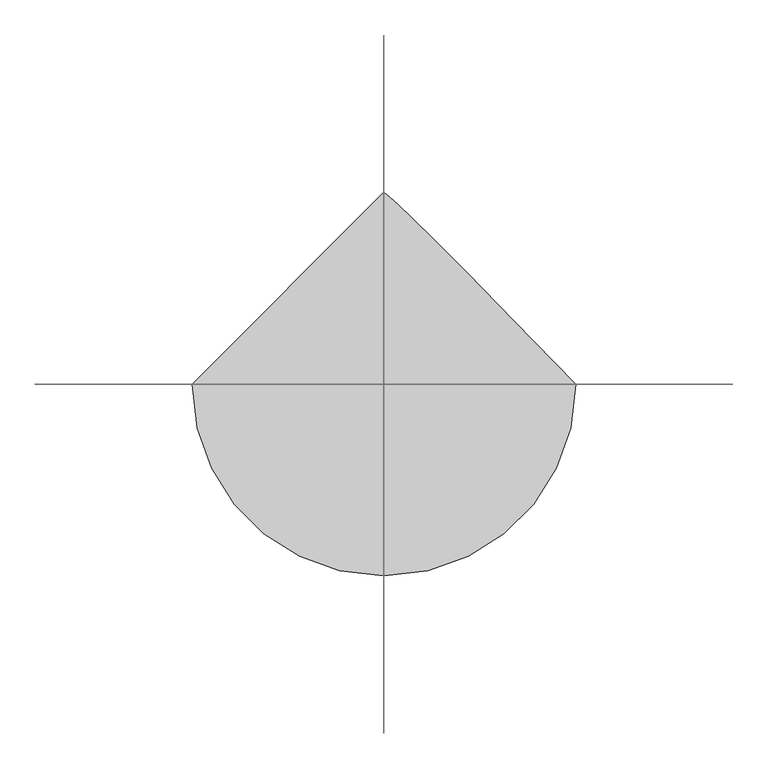
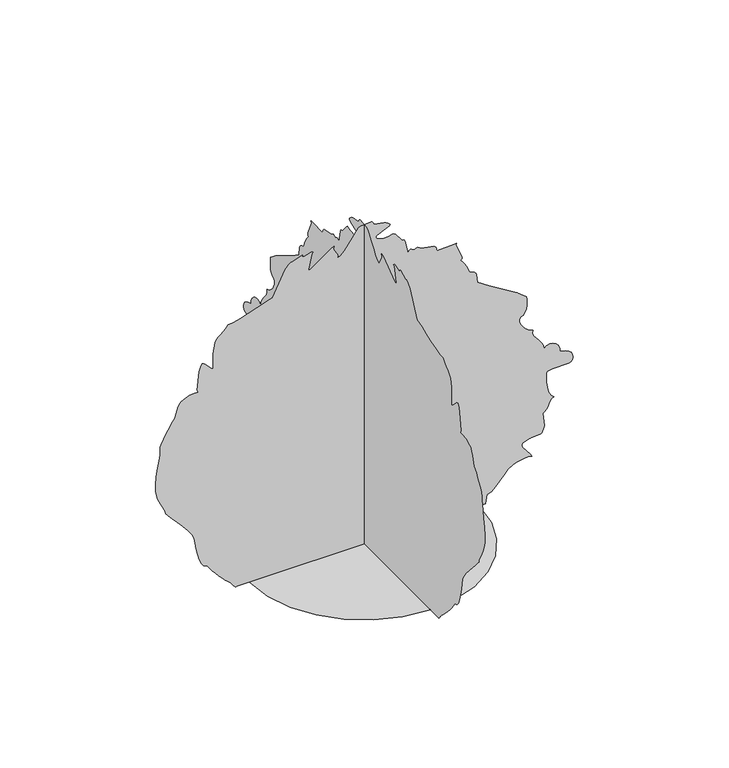
"""IFC4 building model written with IfcOpenShell, lengths in millimetres: proxy geometry, vibernum 26767 : vibernum 26767."""

from ifc_helpers import new_model, si_unit, origin, place, context, project, spatial, triangles, source, transform, mapped, element, save


def entourage_5c4a15e9(model_context):
    return source(origin(), model_context, "Body", "Tessellation", [
        triangles([(-310.4009663, 0.0, 0.0), (-302.1967432, -71.1236111, 0.0), (-278.8261857, -136.4392555, 0.0), (-242.1615087, -194.0757083, 0.0), (-194.0757083, -242.1615087, 0.0), (-136.4392555, -278.8261857, 0.0), (-71.1236111, -302.1967432, 0.0), (1.36e-05, -310.4009663, 0.0), (71.1236111, -302.1967432, 0.0), (136.4392555, -278.8261857, 0.0), (194.0757083, -242.1615087, 0.0), (242.1615087, -194.0757083, 0.0), (278.8261857, -136.4392555, 0.0), (302.1967432, -71.1236111, 0.0), (310.4009663, 2.71e-05, 0.0), (209.5283262, 103.4718092, 0.0), (134.7455816, 179.6535872, 0.0), (81.7052599, 233.0934394, 0.0), (46.0591254, 268.3410517, 0.0), (23.45852, 289.9412231, 0.0), (9.5549798, 302.4456561, 0.0), (-4.07e-05, 310.4009663, 0.0), (-352.7554667, 2.15e-05, 4.3495503), (-355.9965117, 2.13e-05, 8.4826161), (-359.0826241, 2.1e-05, 12.3234041), (-362.0188548, 2.08e-05, 15.7959676), (-364.8077834, 2.07e-05, 18.8245652), (-367.457004, 2.05e-05, 21.3332227), (-369.9665528, 2.04e-05, 23.2460988), (-375.8161594, 2.01e-05, 28.5320975), (-383.5606359, 1.96e-05, 36.3306653), (-392.4582396, 1.9e-05, 45.9079945), (-401.7775108, 1.84e-05, 56.5300297), (-410.7742001, 1.78e-05, 67.463215), (-418.7091808, 1.71e-05, 77.9737471), (-424.8483773, 1.66e-05, 87.3278091), (-434.3200376, 1.64e-05, 90.3102761), (-441.518399, 1.59e-05, 99.1873323), (-446.9133459, 1.51e-05, 112.4136326), (-450.9672046, 1.41e-05, 128.4448579), (-454.1523663, 1.31e-05, 145.7354086), (-456.9311211, 1.21e-05, 162.7404662), (-459.7733894, 1.12e-05, 177.9152122), (-465.8821009, 1.05e-05, 189.8085088), (-476.9463238, 9.6e-06, 205.0848474), (-490.9620744, 8.5e-06, 222.0754346), (-505.927767, 7.5e-06, 239.1112225), (-519.8393452, 6.6e-06, 254.5234358), (-530.6927888, 5.9e-06, 266.6443348), (-536.4840051, 5.5e-06, 273.804599), (-537.980062, 5.1e-06, 279.9056801), (-541.2769901, 4.6e-06, 287.7695352), (-545.6533945, 4.1e-06, 296.6874683), (-550.3904963, 3.6e-06, 305.9584685), (-554.7669371, 3e-06, 314.8764198), (-558.0638288, 2.6e-06, 322.7377496), (-559.5599221, 2.2e-06, 328.8413741), (-564.0633173, 1.1e-06, 346.2505222), (-564.6424607, -1e-07, 367.0963428), (-562.5393188, -1.4e-06, 389.5906094), (-558.9909525, -2.8e-06, 411.9375375), (-555.2393646, -4e-06, 432.3439227), (-552.5215799, -5e-06, 449.0164879), (-552.0770576, -5.6e-06, 460.1619922), (-551.4522048, -6.2e-06, 469.7809908), (-548.1832546, -6.8e-06, 479.8495623), (-543.0422894, -7.4e-06, 490.1772022), (-536.8090942, -8.1e-06, 500.5785295), (-530.2609838, -8.7e-06, 510.8553732), (-524.1776705, -9.2e-06, 520.822352), (-519.3338891, -9.8e-06, 530.2863819), (-514.6958364, -1.01e-05, 534.5764544), (-511.1779552, -1.05e-05, 541.7037083), (-508.3280565, -1.1e-05, 550.5352913), (-505.7042341, -1.16e-05, 559.930757), (-502.8569152, -1.21e-05, 568.7597966), (-499.3364542, -1.25e-05, 575.8870505), (-494.6984015, -1.28e-05, 580.1796301), (-488.7141738, -1.3e-05, 583.3724221), (-483.0575787, -1.32e-05, 586.1308657), (-477.4467293, -1.33e-05, 588.3914835), (-471.5996298, -1.34e-05, 590.0856388), (-465.2318499, -1.35e-05, 591.1448401), (-458.0563431, -1.35e-05, 591.5029578), (-449.7962731, -1.35e-05, 591.0940438), (-452.0898831, -1.38e-05, 597.7844058), (-446.8498687, -1.69e-05, 648.1323137), (-442.8239516, -1.75e-05, 659.7223766), (-438.0639951, -1.8e-05, 668.1551468), (-434.5155925, -1.8e-05, 667.6064884), (-430.9748566, -1.79e-05, 665.0360058), (-414.5257879, -1.68e-05, 647.428723), (-409.2578319, -1.66e-05, 644.4162615), (-408.9962199, -1.74e-05, 657.4007887), (-409.1181238, -1.79e-05, 666.2653639), (-409.3213454, -1.83e-05, 672.7017443), (-409.3035413, -1.87e-05, 678.4040852), (-408.7625133, -1.91e-05, 685.0639257), (-407.3934834, -1.96e-05, 694.3755667), (-404.8915649, -2.04e-05, 708.0306198), (-403.2913719, -2.1e-05, 717.4769182), (-399.8064829, -2.14e-05, 724.3451036), (-394.8255369, -2.17e-05, 729.6460882), (-388.7295427, -2.2e-05, 734.3907841), (-381.9096102, -2.23e-05, 739.5952629), (-374.7468206, -2.27e-05, 746.2703642), (-367.6271971, -2.33e-05, 755.4296162), (-354.5182589, -2.33e-05, 756.2449734), (-335.3386883, -2.36e-05, 761.043009), (-312.9155657, -2.4e-05, 768.2718555), (-290.0885433, -2.45e-05, 776.3821163), (-269.6872632, -2.49e-05, 783.819235), (-254.5437653, -2.53e-05, 789.0313442), (-247.4939957, -2.53e-05, 790.4715179), (-213.6794536, -2.94e-05, 858.769602), (-205.2583288, -3e-05, 869.5493946), (-197.3670409, -3.03e-05, 874.0807314), (-193.2331907, -3.03e-05, 873.8495682), (-168.7295447, -3.09e-05, 884.1188541), (-166.460806, -3.09e-05, 883.4558859), (-168.0742249, -3.06e-05, 879.0896553), (-161.877383, -3.06e-05, 879.3893463), (-144.3734641, -3.09e-05, 884.8376329), (-141.0938133, -3.09e-05, 884.1543898), (-137.9627544, -3.07e-05, 881.4086271), (-140.7920603, -3.07e-05, 880.4332506), (-150.2901451, -2.82e-05, 838.0508085), (-150.4359393, -2.79e-05, 834.0097034), (-142.0369153, -2.81e-05, 837.3624784), (-89.9201382, -3.04e-05, 875.4065952), (-81.5211142, -3.06e-05, 878.7594429), (-83.236371, -3.02e-05, 872.9860308), (-82.0336828, -2.99e-05, 867.6621552), (-72.5891921, -2.9e-05, 852.5922901), (-71.3862495, -2.87e-05, 847.2684872), (-73.1015109, -2.84e-05, 841.495075), (-63.556186, -2.86e-05, 845.6047806), (-53.0855361, -2.92e-05, 856.2092932), (-42.3674857, -3.01e-05, 870.5983858), (-32.0797166, -3.1e-05, 886.0492596), (-22.9007347, -3.19e-05, 899.8541582), (-15.50783, -3.24e-05, 909.2952971), (-10.5790577, -3.25e-05, 911.6575075), (18.9106201, -3.27e-05, 914.4007267), (21.5322068, -3.27e-05, 913.1789989), (23.8564858, -3.25e-05, 909.8845779), (26.6850082, -3.21e-05, 903.8622711), (53.36646, -3.19e-05, 899.8287237), (58.7731068, -3.17e-05, 897.4639698), (63.9669031, -3.15e-05, 893.9232702), (69.0938976, -3.12e-05, 888.8939987), (68.0601171, -3.1e-05, 885.5234196), (63.3263127, -3.08e-05, 882.1706446), (34.7215748, -3.01e-05, 870.0904226), (31.9859905, -2.99e-05, 867.6900604), (32.133565, -2.97e-05, 863.7226427), (35.5686638, -2.95e-05, 860.1538925), (41.5277613, -2.93e-05, 857.2862623), (49.2473392, -2.92e-05, 855.4244574), (57.9630999, -2.92e-05, 854.8808859), (66.9122902, -2.92e-05, 855.9553116), (75.3308715, -2.94e-05, 858.9575993), (79.5358429, -2.94e-05, 858.9905914), (84.1909094, -2.92e-05, 855.1374109), (99.0570351, -2.8e-05, 835.8054514), (103.7123468, -2.78e-05, 831.9522709), (107.9173227, -2.78e-05, 831.9827196), (110.5566329, -2.75e-05, 826.9687815), (117.7400153, -2.54e-05, 791.6018269), (122.069702, -2.57e-05, 796.2169521), (125.2845857, -2.58e-05, 797.6521116), (127.9442162, -2.57e-05, 797.0729319), (133.8415943, -2.56e-05, 794.512623), (138.1999856, -2.56e-05, 794.8580961), (144.2457012, -2.58e-05, 797.8374928), (154.0983702, -2.54e-05, 791.6500797), (188.4892397, -2.5e-05, 784.7844378), (193.5639118, -2.47e-05, 779.5723286), (196.3218285, -2.41e-05, 769.7729994), (243.3426139, -2.42e-05, 771.0379658), (249.3334547, -2.43e-05, 772.2673239), (247.7520468, -2.39e-05, 766.8596598), (263.6852313, -2.17e-05, 729.0644377), (264.3888039, -2.13e-05, 722.3968941), (260.2486133, -2.11e-05, 719.5673429), (264.4396183, -2.09e-05, 715.6404751), (268.5899827, -2.05e-05, 710.080422), (272.58794, -2.02e-05, 703.4306826), (276.3268288, -1.97e-05, 696.2399878), (279.6948645, -1.93e-05, 689.0492203), (282.5828423, -1.89e-05, 682.4020243), (284.8815392, -1.86e-05, 676.8470581), (292.1535699, -1.84e-05, 674.5203833), (297.5205933, -1.82e-05, 671.6629269), (301.2772681, -1.8e-05, 668.0231054), (303.7181983, -1.78e-05, 663.3520243), (306.0880391, -1.64e-05, 640.6748474), (337.5484735, -1.51e-05, 619.285528), (412.8366832, -1.23e-05, 572.7882208), (438.1198783, -1.12e-05, 553.4791523), (439.8826341, -1.08e-05, 546.9589471), (439.9893136, -9.7e-06, 528.3128105), (438.1224217, -9.1e-06, 518.4956772), (434.833124, -8.6e-06, 509.8850836), (430.0172479, -8.2e-06, 503.634157), (423.57073, -8.1e-06, 500.8960247), (419.6083265, -7.7e-06, 495.2673712), (419.9613936, -7.3e-06, 487.2053996), (423.7561475, -6.7e-06, 477.8835849), (430.1112465, -6.1e-06, 468.4703513), (438.1503633, -5.6e-06, 460.136594), (446.9946273, -5.3e-06, 454.0533171), (455.7652765, -5.1e-06, 451.3913793), (454.5663671, -4.6e-06, 443.4767461), (457.9420332, -4.1e-06, 435.1353584), (464.2260246, -3.6e-06, 426.3952306), (471.7495116, -3.1e-06, 417.2791446), (478.8462805, -2.5e-06, 407.8151147), (483.8449943, -1.9e-06, 398.025923), (485.0794393, -1.3e-06, 387.9344968), (492.6181506, -1.7e-06, 394.3632468), (501.3405107, -1.8e-06, 396.5095548), (510.2914905, -1.8e-06, 394.9982735), (518.5109379, -1.5e-06, 390.4541831), (525.0463675, -1.1e-06, 383.5047526), (528.9401705, -5e-07, 374.7773057), (529.2322675, 0.0, 364.8966951), (543.28359, 2e-07, 361.6200783), (553.2505325, 5e-07, 356.9591709), (559.7300789, 8e-07, 351.3864369), (563.3267344, 1.2e-06, 345.3742312), (564.6424607, 1.5e-06, 339.3975975), (564.2741693, 1.9e-06, 333.9264562), (562.8263652, 2.1e-06, 329.438249), (558.5058077, 2.4e-06, 325.0237292), (551.6808246, 2.5e-06, 323.3371679), (508.3052018, 2.5e-06, 323.4667022), (495.6814084, 2.7e-06, 320.1113837), (493.0550426, 3e-06, 315.2853702), (491.9247336, 3.6e-06, 304.683401), (492.3870237, 4.5e-06, 290.5000371), (494.5434691, 5.4e-06, 274.934908), (498.4855614, 6.3e-06, 260.1850997), (504.3148567, 7e-06, 248.4462268), (512.1304407, 7.4e-06, 241.918682), (506.1944658, 7.6e-06, 237.9293542), (502.0110729, 7.9e-06, 232.375896), (498.8894248, 8.3e-06, 225.9143899), (496.1360682, 8.7e-06, 219.2011551), (493.06518, 9.1e-06, 212.8918018), (488.9859595, 9.4e-06, 207.6423766), (483.2074605, 9.6e-06, 204.1089804), (486.5094392, 1.18e-05, 167.9235982), (484.7949363, 1.23e-05, 159.1671923), (479.7174846, 1.29e-05, 149.4257811), (478.0410971, 1.3e-05, 147.3986065), (448.2189348, 1.31e-05, 145.3638107), (427.0784738, 1.35e-05, 138.6241693), (425.673872, 1.39e-05, 132.82763), (427.5890167, 1.42e-05, 126.7778539), (449.1968184, 1.58e-05, 99.5421708), (453.2709884, 1.63e-05, 91.8492719), (446.9844898, 1.62e-05, 94.1108889), (432.729982, 1.62e-05, 94.2706539), (416.3113984, 1.64e-05, 90.1472137), (414.6045259, 1.65e-05, 89.3547294), (401.3177642, 1.66e-05, 85.9130245), (388.9555827, 1.72e-05, 76.9775597), (377.2588766, 1.79e-05, 64.7009653), (365.9660339, 1.87e-05, 51.235649), (354.8103559, 1.95e-05, 38.7350312), (343.5327375, 2e-05, 29.3512471), (331.8716034, 2.03e-05, 25.2371292), (326.9541347, 2.18e-05, 4e-05), (-349.3544025, 2.18e-05, 4e-05), (-4.6e-06, -352.7554667, 4.3495758), (-4.6e-06, -355.9965117, 8.4826416), (-4.6e-06, -359.0826241, 12.3234041), (-4.6e-06, -362.0188548, 15.7959937), (-4.6e-06, -364.8077834, 18.8245902), (-4.6e-06, -367.457004, 21.3332477), (-4.6e-06, -369.9665528, 23.2460988), (-4.6e-06, -375.8161594, 28.5320975), (-4.6e-06, -383.5606359, 36.3306653), (-4.6e-06, -392.4582396, 45.9079945), (-4.6e-06, -401.7775108, 56.5300297), (-4.6e-06, -410.7742001, 67.4634693), (-4.6e-06, -418.7091808, 77.9737471), (-4.6e-06, -424.8483773, 87.3278091), (-4.6e-06, -434.3200376, 90.3102761), (-4.6e-06, -441.518399, 99.1873323), (-4.6e-06, -446.9133459, 112.4138869), (-4.6e-06, -450.9672046, 128.4448579), (-4.6e-06, -454.1523663, 145.7354086), (-4.6e-06, -456.9311211, 162.7404662), (-4.6e-06, -459.7733894, 177.9152122), (-4.6e-06, -465.8821009, 189.8085088), (-4.6e-06, -476.9463238, 205.0848474), (-4.6e-06, -490.9620744, 222.0754346), (-4.6e-06, -505.927767, 239.1112225), (-4.6e-06, -519.8393452, 254.5234358), (-4.6e-06, -530.6927888, 266.6443348), (-4.6e-06, -536.4840051, 273.804599), (-4.6e-06, -537.980062, 279.9056801), (-4.6e-06, -541.2769901, 287.7695352), (-4.6e-06, -545.6533945, 296.6874683), (-4.6e-06, -550.3904963, 305.9584685), (-4.6e-06, -554.7669371, 314.8764198), (-4.6e-06, -558.0638288, 322.7377496), (-4.6e-06, -559.5599221, 328.8413741), (-4.6e-06, -564.0633173, 346.2505222), (-4.6e-06, -564.6424607, 367.0963428), (-4.6e-06, -562.5393188, 389.5906094), (-4.6e-06, -558.9909525, 411.9375375), (-4.6e-06, -555.2393646, 432.3439227), (-4.6e-06, -552.5215799, 449.0164879), (-4.6e-06, -552.0770576, 460.1619922), (-4.6e-06, -551.4522048, 469.7809908), (-4.6e-06, -548.1832546, 479.8495623), (-4.6e-06, -543.0422894, 490.1772022), (-4.6e-06, -536.8090942, 500.5785295), (-4.6e-06, -530.2609838, 510.8553732), (-4.6e-06, -524.1776705, 520.822352), (-4.6e-06, -519.3338891, 530.2863819), (-4.6e-06, -514.6958364, 534.5764544), (-4.6e-06, -511.1779552, 541.7037083), (-4.6e-06, -508.3280565, 550.5352913), (-4.6e-06, -505.7042341, 559.930757), (-4.6e-06, -502.8569152, 568.7597966), (-4.6e-06, -499.3364542, 575.889594), (-4.6e-06, -494.6984015, 580.1796301), (-4.6e-06, -488.7141738, 583.3724221), (-4.6e-06, -483.0575787, 586.1308657), (-4.6e-06, -477.4467293, 588.3914835), (-4.6e-06, -471.5996298, 590.0856388), (-4.6e-06, -465.2318499, 591.1448401), (-4.6e-06, -458.0563431, 591.5029578), (-4.6e-06, -449.7962731, 591.0940438), (-4.6e-06, -452.0898831, 597.7844058), (-4.6e-06, -446.8498687, 648.1323137), (-4.6e-06, -442.8239516, 659.7223766), (-4.6e-06, -438.0639951, 668.1551468), (-4.6e-06, -434.5155925, 667.6064884), (-4.6e-06, -430.9748566, 665.0360058), (-4.6e-06, -414.5257879, 647.428723), (-4.6e-06, -409.2578319, 644.4162615), (-4.6e-06, -408.9962199, 657.4007887), (-4.6e-06, -409.1181238, 666.2653639), (-4.6e-06, -409.3213454, 672.7017443), (-4.6e-06, -409.3035413, 678.4040852), (-4.6e-06, -408.7625133, 685.0639257), (-4.6e-06, -407.3934834, 694.3755667), (-4.6e-06, -404.8915649, 708.0306198), (-4.6e-06, -403.2913719, 717.4769182), (-4.6e-06, -399.8064829, 724.3451036), (-4.6e-06, -394.8255369, 729.6460882), (-4.6e-06, -388.7295427, 734.3907841), (-4.6e-06, -381.9096102, 739.5952629), (-4.6e-06, -374.7468206, 746.2703642), (-4.6e-06, -367.6271971, 755.4296162), (-4.6e-06, -354.5182589, 756.2449734), (-4.6e-06, -335.3386883, 761.043009), (-4.6e-06, -312.9155657, 768.2718555), (-4.6e-06, -290.0885433, 776.3821163), (-4.6e-06, -269.6872632, 783.819235), (-4.6e-06, -254.5437653, 789.0313442), (-4.6e-06, -247.4939957, 790.4715179), (-4.6e-06, -213.6794536, 858.769602), (-4.6e-06, -205.2583288, 869.5493946), (-4.6e-06, -197.3670409, 874.0807314), (-4.6e-06, -193.2331907, 873.8495682), (-4.6e-06, -168.7295447, 884.1188541), (-4.6e-06, -166.4605516, 883.4558859), (-4.6e-06, -168.0742249, 879.0896553), (-4.6e-06, -161.877383, 879.3893463), (-4.6e-06, -144.3734641, 884.8376329), (-4.6e-06, -141.0938133, 884.1543898), (-4.6e-06, -137.9627544, 881.4086271), (-4.6e-06, -140.7920603, 880.4332506), (-4.6e-06, -150.2901451, 838.0508085), (-4.6e-06, -150.4359393, 834.0121742), (-4.6e-06, -142.0369153, 837.3624784), (-4.6e-06, -89.9201382, 875.4065952), (-4.6e-06, -81.5211142, 878.7594429), (-4.6e-06, -83.236371, 872.9860308), (-4.6e-06, -82.0336828, 867.6621552), (-4.6e-06, -72.5891921, 852.5922901), (-4.6e-06, -71.3862495, 847.2684872), (-4.6e-06, -73.1015109, 841.495075), (-4.6e-06, -63.556186, 845.6047806), (-4.6e-06, -53.0855361, 856.2092932), (-4.6e-06, -42.3674857, 870.5983858), (-4.6e-06, -32.0797166, 886.0492596), (-4.6e-06, -22.9007347, 899.8541582), (-4.6e-06, -15.50783, 909.2952971), (-4.6e-06, -10.5790577, 911.6575075), (-4.6e-06, 18.9106201, 914.4007267), (-4.6e-06, 21.5322068, 913.1789989), (-4.6e-06, 23.8564858, 909.8845779), (-4.6e-06, 26.6850082, 903.8622711), (-4.6e-06, 53.36646, 899.8287237), (-4.6e-06, 58.7731068, 897.4639698), (-4.6e-06, 63.9669031, 893.9232702), (-4.6e-06, 69.0938976, 888.8939987), (-4.6e-06, 68.0601171, 885.5234196), (-4.6e-06, 63.3263127, 882.173188), (-4.6e-06, 34.7215748, 870.0904226), (-4.6e-06, 31.9859905, 867.6900604), (-4.6e-06, 32.133565, 863.7226427), (-4.6e-06, 35.5686638, 860.1538925), (-4.6e-06, 41.5277613, 857.2862623), (-4.6e-06, 49.2473392, 855.4269281), (-4.6e-06, 57.9630999, 854.8808859), (-4.6e-06, 66.9122902, 855.9553116), (-4.6e-06, 75.3308715, 858.9575993), (-4.6e-06, 79.5358429, 858.9905914), (-4.6e-06, 84.1909094, 855.1374109), (-4.6e-06, 99.0570351, 835.8054514), (-4.6e-06, 103.7123468, 831.9522709), (-4.6e-06, 107.9173227, 831.9852631), (-4.6e-06, 110.5566329, 826.9687815), (-4.6e-06, 117.7400153, 791.6018269), (-4.6e-06, 122.069702, 796.2169521), (-4.6e-06, 125.2845857, 797.6521116), (-4.6e-06, 127.9442162, 797.0729319), (-4.6e-06, 133.8415943, 794.512623), (-4.6e-06, 138.1999856, 794.8580961), (-4.6e-06, 144.2457012, 797.8374928), (-4.6e-06, 154.0983702, 791.6500797), (-4.6e-06, 188.4892397, 784.7844378), (-4.6e-06, 193.5639118, 779.5723286), (-4.6e-06, 196.3218285, 769.7729994), (-4.6e-06, 243.3426139, 771.0379658), (-4.6e-06, 249.3334547, 772.2673239), (-4.6e-06, 247.7520468, 766.8596598), (-4.6e-06, 263.6852313, 729.0644377), (-4.6e-06, 264.3888039, 722.3968941), (-4.6e-06, 260.2486133, 719.5673429), (-4.6e-06, 264.4396183, 715.6404751), (-4.6e-06, 268.5899827, 710.080422), (-4.6e-06, 272.58794, 703.4306826), (-4.6e-06, 276.3268288, 696.2399878), (-4.6e-06, 279.6948645, 689.0492203), (-4.6e-06, 282.5828423, 682.4020243), (-4.6e-06, 284.8815392, 676.8470581), (-4.6e-06, 292.1535699, 674.5203833), (-4.6e-06, 297.5205933, 671.6629269), (-4.6e-06, 301.2772681, 668.0231054), (-4.6e-06, 303.7181983, 663.3520243), (-4.6e-06, 306.0880391, 640.6748474), (-4.6e-06, 337.5484735, 619.285528), (-4.6e-06, 412.8366832, 572.7907642), (-4.6e-06, 438.1198783, 553.4791523), (-4.6e-06, 439.8826341, 546.9589471), (-4.6e-06, 439.9893136, 528.3128105), (-4.6e-06, 438.1224217, 518.4956772), (-4.6e-06, 434.833124, 509.8850836), (-4.6e-06, 430.0172479, 503.634157), (-4.6e-06, 423.57073, 500.8960247), (-4.6e-06, 419.6083265, 495.2673712), (-4.6e-06, 419.9613936, 487.2053996), (-4.6e-06, 423.7561475, 477.8835849), (-4.6e-06, 430.1112465, 468.4703513), (-4.6e-06, 438.1503633, 460.136594), (-4.6e-06, 446.9946273, 454.0533171), (-4.6e-06, 455.7652765, 451.3913793), (-4.6e-06, 454.5663671, 443.4767461), (-4.6e-06, 457.9420332, 435.1353584), (-4.6e-06, 464.2260246, 426.3952306), (-4.6e-06, 471.7495116, 417.2791446), (-4.6e-06, 478.8462805, 407.8151147), (-4.6e-06, 483.8449943, 398.025923), (-4.6e-06, 485.0794393, 387.9344968), (-4.6e-06, 492.6181506, 394.3632468), (-4.6e-06, 501.3405107, 396.5095548), (-4.6e-06, 510.2914905, 394.9982735), (-4.6e-06, 518.5109379, 390.4541831), (-4.6e-06, 525.0463675, 383.5047526), (-4.6e-06, 528.9401705, 374.7773057), (-4.6e-06, 529.2322675, 364.8966951), (-4.6e-06, 543.28359, 361.6200783), (-4.6e-06, 553.2505325, 356.9591709), (-4.6e-06, 559.7300789, 351.3864369), (-4.6e-06, 563.3267344, 345.3742312), (-4.6e-06, 564.6424607, 339.3975975), (-4.6e-06, 564.2741693, 333.9264562), (-4.6e-06, 562.8263652, 329.438249), (-4.6e-06, 558.5058077, 325.0237292), (-4.6e-06, 551.6808246, 323.3371679), (-4.6e-06, 508.3052018, 323.4667022), (-4.6e-06, 495.6814084, 320.1113837), (-4.6e-06, 493.0550426, 315.2853702), (-4.6e-06, 491.9247336, 304.683401), (-4.6e-06, 492.3870237, 290.5000371), (-4.6e-06, 494.5434691, 274.934908), (-4.6e-06, 498.4855614, 260.1850997), (-4.6e-06, 504.3148567, 248.4464812), (-4.6e-06, 512.1304407, 241.918682), (-4.6e-06, 506.1944658, 237.9293542), (-4.6e-06, 502.0110729, 232.375896), (-4.6e-06, 498.8894248, 225.9143899), (-4.6e-06, 496.1360682, 219.2011551), (-4.6e-06, 493.06518, 212.8918018), (-4.6e-06, 488.9859595, 207.6423766), (-4.6e-06, 483.2074605, 204.1089804), (-4.6e-06, 486.5094392, 167.9235982), (-4.6e-06, 484.7949363, 159.1671923), (-4.6e-06, 479.7174846, 149.4257811), (-4.6e-06, 478.0410971, 147.3988609), (-4.6e-06, 448.2189348, 145.3638107), (-4.6e-06, 427.0784738, 138.6241693), (-4.6e-06, 425.673872, 132.8278843), (-4.6e-06, 427.5890167, 126.7778539), (-4.6e-06, 449.1968184, 99.5421708), (-4.6e-06, 453.2709884, 91.8492719), (-4.6e-06, 446.9844898, 94.1108889), (-4.6e-06, 432.729982, 94.2706539), (-4.6e-06, 416.3113984, 90.1472137), (-4.6e-06, 414.6045259, 89.3547294), (-4.6e-06, 401.3177642, 85.9130245), (-4.6e-06, 388.9555827, 76.9775597), (-4.6e-06, 377.2588766, 64.7009653), (-4.6e-06, 365.9660339, 51.235649), (-4.6e-06, 354.8103559, 38.7350312), (-4.6e-06, 343.5327375, 29.3512471), (-4.6e-06, 331.8716034, 25.2371564), (-4.6e-06, 326.9541347, 6.03e-05), (-4.6e-06, -349.3544025, 6.03e-05)], [[21, 22, 1], [20, 21, 1], [19, 20, 1], [18, 19, 1], [17, 18, 1], [17, 1, 2], [17, 2, 3], [17, 3, 4], [16, 17, 4], [16, 4, 5], [16, 5, 6], [16, 6, 7], [16, 7, 8], [16, 8, 9], [16, 9, 10], [16, 10, 11], [16, 11, 12], [15, 16, 12], [14, 15, 12], [13, 14, 12], [261, 262, 263], [130, 131, 132], [124, 125, 126], [180, 181, 182], [244, 245, 246], [119, 120, 121], [118, 119, 121], [212, 213, 214], [273, 274, 275], [123, 124, 126], [260, 261, 263], [88, 89, 90], [88, 90, 91], [260, 263, 264], [87, 88, 91], [87, 91, 92], [122, 123, 126], [166, 167, 168], [150, 151, 152], [150, 152, 153], [149, 150, 153], [148, 149, 153], [148, 153, 154], [147, 148, 154], [147, 154, 155], [87, 92, 93], [183, 184, 185], [122, 126, 127], [121, 122, 127], [174, 175, 176], [130, 132, 133], [129, 130, 133], [260, 264, 265], [129, 133, 134], [129, 134, 135], [129, 135, 136], [273, 275, 23], [86, 87, 93], [85, 86, 93], [273, 23, 24], [273, 24, 25], [273, 25, 26], [118, 121, 127], [118, 127, 128], [106, 107, 108], [273, 26, 27], [260, 265, 266], [260, 266, 267], [259, 260, 267], [244, 246, 247], [179, 180, 182], [273, 27, 28], [255, 256, 257], [162, 163, 164], [161, 162, 164], [117, 118, 128], [116, 117, 128], [115, 116, 128], [114, 115, 128], [273, 28, 29], [273, 29, 30], [273, 30, 31], [273, 31, 32], [273, 32, 33], [273, 33, 34], [273, 34, 35], [273, 35, 36], [161, 164, 165], [170, 171, 172], [169, 170, 172], [169, 172, 173], [254, 255, 257], [253, 254, 257], [252, 253, 257], [252, 257, 258], [243, 244, 247], [160, 161, 165], [36, 37, 38], [243, 247, 248], [36, 38, 39], [273, 36, 39], [273, 39, 40], [273, 40, 41], [273, 41, 42], [273, 42, 43], [273, 43, 44], [273, 44, 45], [273, 45, 46], [273, 46, 47], [272, 273, 47], [271, 272, 47], [270, 271, 47], [269, 270, 47], [268, 269, 47], [267, 268, 47], [259, 267, 47], [258, 259, 47], [252, 258, 47], [252, 47, 48], [252, 48, 49], [252, 49, 50], [252, 50, 51], [252, 51, 52], [252, 52, 53], [252, 53, 54], [252, 54, 55], [252, 55, 56], [252, 56, 57], [252, 57, 58], [252, 58, 59], [252, 59, 60], [252, 60, 61], [252, 61, 62], [252, 62, 63], [252, 63, 64], [252, 64, 65], [252, 65, 66], [252, 66, 67], [252, 67, 68], [252, 68, 69], [252, 69, 70], [252, 70, 71], [252, 71, 72], [252, 72, 73], [252, 73, 74], [252, 74, 75], [252, 75, 76], [252, 76, 77], [252, 77, 78], [252, 78, 79], [252, 79, 80], [252, 80, 81], [252, 81, 82], [252, 82, 83], [252, 83, 84], [252, 84, 85], [252, 85, 93], [252, 93, 94], [252, 94, 95], [252, 95, 96], [252, 96, 97], [252, 97, 98], [252, 98, 99], [252, 99, 100], [252, 100, 101], [252, 101, 102], [252, 102, 103], [252, 103, 104], [252, 104, 105], [252, 105, 106], [252, 106, 108], [252, 108, 109], [252, 109, 110], [252, 110, 111], [252, 111, 112], [252, 112, 113], [252, 113, 114], [252, 114, 128], [252, 128, 129], [252, 129, 136], [252, 136, 137], [252, 137, 138], [251, 252, 138], [250, 251, 138], [249, 250, 138], [248, 249, 138], [243, 248, 138], [242, 243, 138], [241, 242, 138], [240, 241, 138], [239, 240, 138], [238, 239, 138], [238, 138, 139], [238, 139, 140], [238, 140, 141], [238, 141, 142], [238, 142, 143], [237, 238, 143], [234, 235, 236], [233, 234, 236], [232, 233, 236], [231, 232, 236], [230, 231, 236], [229, 230, 236], [228, 229, 236], [227, 228, 236], [227, 236, 237], [179, 182, 183], [179, 183, 185], [199, 200, 201], [199, 201, 202], [199, 202, 203], [199, 203, 204], [199, 204, 205], [199, 205, 206], [199, 206, 207], [198, 199, 207], [198, 207, 208], [144, 145, 146], [144, 146, 147], [144, 147, 155], [143, 144, 155], [143, 155, 156], [237, 143, 156], [237, 156, 157], [237, 157, 158], [237, 158, 159], [237, 159, 160], [177, 178, 179], [226, 227, 237], [225, 226, 237], [224, 225, 237], [223, 224, 237], [222, 223, 237], [221, 222, 237], [220, 221, 237], [220, 237, 160], [219, 220, 160], [218, 219, 160], [166, 168, 169], [165, 166, 169], [160, 165, 169], [218, 160, 169], [217, 218, 169], [216, 217, 169], [215, 216, 169], [215, 169, 173], [215, 173, 174], [215, 174, 176], [211, 212, 214], [211, 214, 215], [194, 195, 196], [193, 194, 196], [192, 193, 196], [192, 196, 197], [197, 198, 208], [176, 177, 179], [197, 208, 209], [176, 179, 185], [185, 186, 187], [176, 185, 187], [176, 187, 188], [176, 188, 189], [176, 189, 190], [176, 190, 191], [176, 191, 192], [176, 192, 197], [176, 197, 209], [176, 209, 210], [215, 176, 210], [211, 215, 210], [514, 515, 516], [383, 384, 385], [377, 378, 379], [433, 434, 435], [497, 498, 499], [372, 373, 374], [371, 372, 374], [465, 466, 467], [526, 527, 528], [376, 377, 379], [513, 514, 516], [341, 342, 343], [341, 343, 344], [513, 516, 517], [340, 341, 344], [340, 344, 345], [375, 376, 379], [419, 420, 421], [403, 404, 405], [403, 405, 406], [402, 403, 406], [401, 402, 406], [401, 406, 407], [400, 401, 407], [400, 407, 408], [340, 345, 346], [436, 437, 438], [375, 379, 380], [374, 375, 380], [427, 428, 429], [383, 385, 386], [382, 383, 386], [513, 517, 518], [382, 386, 387], [382, 387, 388], [382, 388, 389], [526, 528, 276], [339, 340, 346], [338, 339, 346], [526, 276, 277], [526, 277, 278], [526, 278, 279], [371, 374, 380], [371, 380, 381], [359, 360, 361], [526, 279, 280], [513, 518, 519], [513, 519, 520], [512, 513, 520], [497, 499, 500], [432, 433, 435], [526, 280, 281], [508, 509, 510], [415, 416, 417], [414, 415, 417], [370, 371, 381], [369, 370, 381], [368, 369, 381], [367, 368, 381], [526, 281, 282], [526, 282, 283], [526, 283, 284], [526, 284, 285], [526, 285, 286], [526, 286, 287], [526, 287, 288], [526, 288, 289], [414, 417, 418], [423, 424, 425], [422, 423, 425], [422, 425, 426], [507, 508, 510], [506, 507, 510], [505, 506, 510], [505, 510, 511], [496, 497, 500], [413, 414, 418], [289, 290, 291], [496, 500, 501], [289, 291, 292], [526, 289, 292], [526, 292, 293], [526, 293, 294], [526, 294, 295], [526, 295, 296], [526, 296, 297], [526, 297, 298], [526, 298, 299], [526, 299, 300], [525, 526, 300], [524, 525, 300], [523, 524, 300], [522, 523, 300], [521, 522, 300], [520, 521, 300], [512, 520, 300], [511, 512, 300], [505, 511, 300], [505, 300, 301], [505, 301, 302], [505, 302, 303], [505, 303, 304], [505, 304, 305], [505, 305, 306], [505, 306, 307], [505, 307, 308], [505, 308, 309], [505, 309, 310], [505, 310, 311], [505, 311, 312], [505, 312, 313], [505, 313, 314], [505, 314, 315], [505, 315, 316], [505, 316, 317], [505, 317, 318], [505, 318, 319], [505, 319, 320], [505, 320, 321], [505, 321, 322], [505, 322, 323], [505, 323, 324], [505, 324, 325], [505, 325, 326], [505, 326, 327], [505, 327, 328], [505, 328, 329], [505, 329, 330], [505, 330, 331], [505, 331, 332], [505, 332, 333], [505, 333, 334], [505, 334, 335], [505, 335, 336], [505, 336, 337], [505, 337, 338], [505, 338, 346], [505, 346, 347], [505, 347, 348], [505, 348, 349], [505, 349, 350], [505, 350, 351], [505, 351, 352], [505, 352, 353], [505, 353, 354], [505, 354, 355], [505, 355, 356], [505, 356, 357], [505, 357, 358], [505, 358, 359], [505, 359, 361], [505, 361, 362], [505, 362, 363], [505, 363, 364], [505, 364, 365], [505, 365, 366], [505, 366, 367], [505, 367, 381], [505, 381, 382], [505, 382, 389], [505, 389, 390], [505, 390, 391], [504, 505, 391], [503, 504, 391], [502, 503, 391], [501, 502, 391], [496, 501, 391], [495, 496, 391], [494, 495, 391], [493, 494, 391], [492, 493, 391], [491, 492, 391], [491, 391, 392], [491, 392, 393], [491, 393, 394], [491, 394, 395], [491, 395, 396], [490, 491, 396], [487, 488, 489], [486, 487, 489], [485, 486, 489], [484, 485, 489], [483, 484, 489], [482, 483, 489], [481, 482, 489], [480, 481, 489], [480, 489, 490], [432, 435, 436], [432, 436, 438], [452, 453, 454], [452, 454, 455], [452, 455, 456], [452, 456, 457], [452, 457, 458], [452, 458, 459], [452, 459, 460], [451, 452, 460], [451, 460, 461], [397, 398, 399], [397, 399, 400], [397, 400, 408], [396, 397, 408], [396, 408, 409], [490, 396, 409], [490, 409, 410], [490, 410, 411], [490, 411, 412], [490, 412, 413], [430, 431, 432], [479, 480, 490], [478, 479, 490], [477, 478, 490], [476, 477, 490], [475, 476, 490], [474, 475, 490], [473, 474, 490], [473, 490, 413], [472, 473, 413], [471, 472, 413], [419, 421, 422], [418, 419, 422], [413, 418, 422], [471, 413, 422], [470, 471, 422], [469, 470, 422], [468, 469, 422], [468, 422, 426], [468, 426, 427], [468, 427, 429], [464, 465, 467], [464, 467, 468], [447, 448, 449], [446, 447, 449], [445, 446, 449], [445, 449, 450], [450, 451, 461], [429, 430, 432], [450, 461, 462], [429, 432, 438], [438, 439, 440], [429, 438, 440], [429, 440, 441], [429, 441, 442], [429, 442, 443], [429, 443, 444], [429, 444, 445], [429, 445, 450], [429, 450, 462], [429, 462, 463], [468, 429, 463], [464, 468, 463]], closed=False),
    ])


if __name__ == "__main__":
    model = new_model("IFC4")
    model_context = context("Model", 3, world=origin())
    ifc_project = project(units=[si_unit("LENGTHUNIT", "METRE", prefix="MILLI")], contexts=[model_context])
    site = spatial("IfcSite", under=ifc_project)
    building = spatial("IfcBuilding", under=site)
    placement = place(None, origin())
    entourage_shape = entourage_5c4a15e9(model_context)
    element("IfcBuildingElementProxy", 1, Name="vibernum 26767 : vibernum 26767", ObjectType="vibernum 26767 : vibernum 26767", at=placement, inside=building, context=model_context, shape_type="MappedRepresentation", body=[
        mapped(entourage_shape, transform((0.0, 0.0, 0.0), x_axis=(1.0, 0.0, 0.0), y_axis=(0.0, 1.0, 0.0), z_axis=(0.0, 0.0, 1.0))),
    ])
    save(model, "model.ifc")

# Revit data of these elements
# Type "vibernum 26767 : vibernum 26767"
#   built-in parameter 1005195 = "RPC-16-FU5P-8RFX-7Q0N-4000-ST1L-LVER-AU"
#   Height = 0
